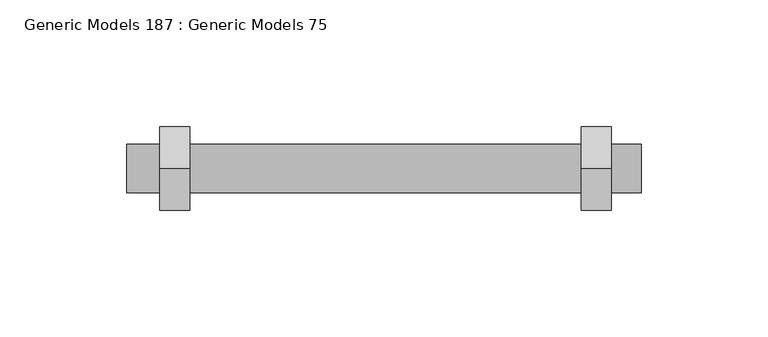
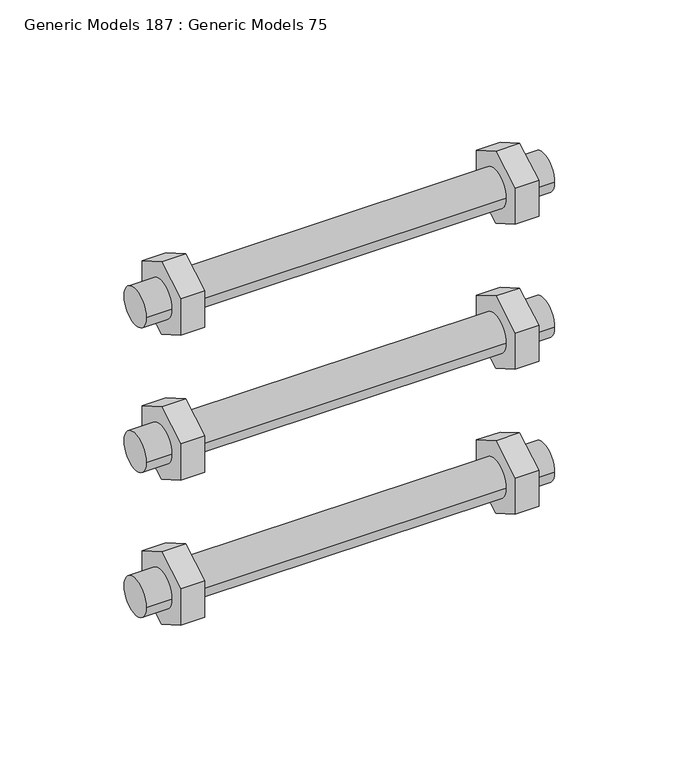
"""IFC4 building model written with IfcOpenShell, lengths in millimetres: proxy geometry, Generic Models 187 : Generic Models 75."""

from ifc_helpers import new_model, si_unit, point, frame, frame_2d, origin, place, context, project, spatial, polyline, circle_curve, trimmed, segment, composite_curve, outline, extrude, source, transform, mapped, element, save


def generic_models_187_generic_models_75_f4eb34d6(model_context):
    return source(origin(), model_context, "Body", "SweptSolid", [
        extrude(outline(polyline([(35157.8873281, 271852.097122), (35157.8873281, 271833.047122), (35141.3895442, 271823.522122), (35124.8917603, 271833.047122), (35124.8917603, 271852.097122), (35141.3895442, 271861.622122), (35157.8873281, 271852.097122)])), frame((31918.2596032, 0.0, 0.0), z_axis=(1.0, 0.0, 0.0), x_axis=(0.0, 1.0, 0.0)), (0.0, 0.0, 1.0), 11.90625),
        extrude(outline(polyline([(35157.8873281, 271775.897122), (35157.8873281, 271756.847122), (35141.3895442, 271747.322122), (35124.8917603, 271756.847122), (35124.8917603, 271775.897122), (35141.3895442, 271785.422122), (35157.8873281, 271775.897122)])), frame((31918.2596032, 0.0, 0.0), z_axis=(1.0, 0.0, 0.0), x_axis=(0.0, 1.0, 0.0)), (0.0, 0.0, 1.0), 11.90625),
        extrude(outline(polyline([(35157.8873281, 271699.697122), (35157.8873281, 271680.647122), (35141.3895442, 271671.122122), (35124.8917603, 271680.647122), (35124.8917603, 271699.697122), (35141.3895442, 271709.222122), (35157.8873281, 271699.697122)])), frame((31918.2596032, 0.0, 0.0), z_axis=(1.0, 0.0, 0.0), x_axis=(0.0, 1.0, 0.0)), (0.0, 0.0, 1.0), 11.90625),
        extrude(outline(polyline([(35157.8873281, 271852.097122), (35157.8873281, 271833.047122), (35141.3895442, 271823.522122), (35124.8917603, 271833.047122), (35124.8917603, 271852.097122), (35141.3895442, 271861.622122), (35157.8873281, 271852.097122)])), frame((31751.9689782, 0.0, 0.0), z_axis=(1.0, 0.0, 0.0), x_axis=(0.0, 1.0, 0.0)), (0.0, 0.0, 1.0), 11.90625),
        extrude(outline(polyline([(35157.8873281, 271775.897122), (35157.8873281, 271756.847122), (35141.3895442, 271747.322122), (35124.8917603, 271756.847122), (35124.8917603, 271775.897122), (35141.3895442, 271785.422122), (35157.8873281, 271775.897122)])), frame((31751.9689782, 0.0, 0.0), z_axis=(1.0, 0.0, 0.0), x_axis=(0.0, 1.0, 0.0)), (0.0, 0.0, 1.0), 11.90625),
        extrude(outline(polyline([(35157.8873281, 271699.697122), (35157.8873281, 271680.647122), (35141.3895442, 271671.122122), (35124.8917603, 271680.647122), (35124.8917603, 271699.697122), (35141.3895442, 271709.222122), (35157.8873281, 271699.697122)])), frame((31751.9689782, 0.0, 0.0), z_axis=(1.0, 0.0, 0.0), x_axis=(0.0, 1.0, 0.0)), (0.0, 0.0, 1.0), 11.90625),
        extrude(outline(composite_curve([segment(trimmed(circle_curve(frame_2d((35141.3895442, 271766.372122)), 9.525), [point((35131.8645442, 271766.372122))], [point((35150.9145442, 271766.372122))], False, "CARTESIAN"), True, "CONTINUOUS"), segment(trimmed(circle_curve(frame_2d((35141.3895442, 271766.372122)), 9.525), [point((35150.9145442, 271766.372122))], [point((35131.8645442, 271766.372122))], False, "CARTESIAN"), True, "CONTINUOUS")], self_intersect=False)), frame((31738.8721032, 0.0, 0.0), z_axis=(1.0, 0.0, 0.0), x_axis=(0.0, 1.0, 0.0)), (0.0, 0.0, 1.0), 203.2),
        extrude(outline(composite_curve([segment(trimmed(circle_curve(frame_2d((35141.3895442, 271690.172122)), 9.525), [point((35131.8645442, 271690.172122))], [point((35150.9145442, 271690.172122))], False, "CARTESIAN"), True, "CONTINUOUS"), segment(trimmed(circle_curve(frame_2d((35141.3895442, 271690.172122)), 9.525), [point((35150.9145442, 271690.172122))], [point((35131.8645442, 271690.172122))], False, "CARTESIAN"), True, "CONTINUOUS")], self_intersect=False)), frame((31738.8721032, 0.0, 0.0), z_axis=(1.0, 0.0, 0.0), x_axis=(0.0, 1.0, 0.0)), (0.0, 0.0, 1.0), 203.2),
        extrude(outline(composite_curve([segment(trimmed(circle_curve(frame_2d((35141.3895442, 271842.572122)), 9.525), [point((35131.8645442, 271842.572122))], [point((35150.9145442, 271842.572122))], False, "CARTESIAN"), True, "CONTINUOUS"), segment(trimmed(circle_curve(frame_2d((35141.3895442, 271842.572122)), 9.525), [point((35150.9145442, 271842.572122))], [point((35131.8645442, 271842.572122))], False, "CARTESIAN"), True, "CONTINUOUS")], self_intersect=False)), frame((31738.8721032, 0.0, 0.0), z_axis=(1.0, 0.0, 0.0), x_axis=(0.0, 1.0, 0.0)), (0.0, 0.0, 1.0), 203.2),
    ])


if __name__ == "__main__":
    model = new_model("IFC4")
    model_context = context("Model", 3, world=origin())
    ifc_project = project(units=[si_unit("LENGTHUNIT", "METRE", prefix="MILLI")], contexts=[model_context])
    site = spatial("IfcSite", under=ifc_project)
    building = spatial("IfcBuilding", under=site)
    placement = place(None, origin())
    generic_models_187_generic_models_75_shape = generic_models_187_generic_models_75_f4eb34d6(model_context)
    element("IfcBuildingElementProxy", 1, Name="Generic Models 187 : Generic Models 75", ObjectType="Generic Models 187 : Generic Models 75", at=placement, inside=building, context=model_context, shape_type="MappedRepresentation", body=[
        mapped(generic_models_187_generic_models_75_shape, transform((0.0, 0.0, 0.0), x_axis=(1.0, 0.0, 0.0), y_axis=(0.0, 1.0, 0.0), z_axis=(0.0, 0.0, 1.0))),
    ])
    save(model, "model.ifc")
